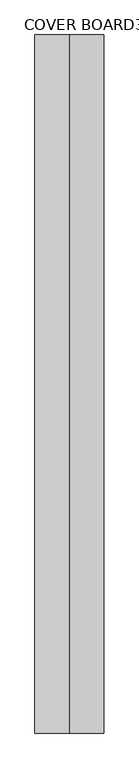
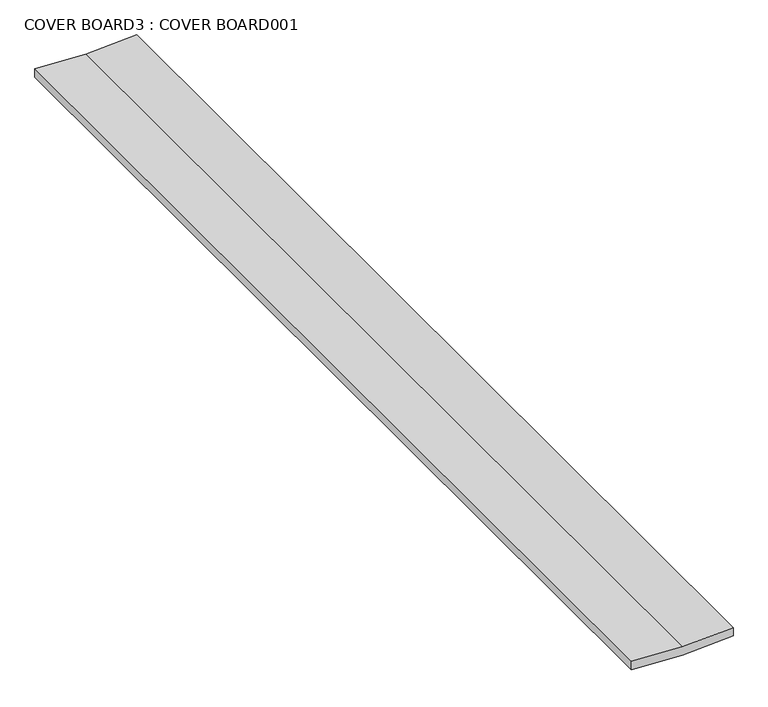
"""IFC4 building model written with IfcOpenShell, lengths in millimetres: proxy geometry, COVER BOARD3 : COVER BOARD001."""

from ifc_helpers import new_model, si_unit, frame, origin, place, context, project, spatial, polyline, outline, extrude, source, transform, mapped, element, save


def cover_board3_cover_board001_2390c736(model_context):
    return source(origin(), model_context, "Body", "SweptSolid", [
        extrude(outline(polyline([(40228.3444286, -4699.8063764), (40233.346, -4797.9038825), (40216.0142809, -4797.9038825), (40211.0127094, -4699.8063764), (40216.0142809, -4601.0538825), (40233.346, -4601.0538825), (40228.3444286, -4699.8063764)])), frame((0.0, -1052.6406573, 0.0), z_axis=(0.0, 1.0, 0.0), x_axis=(0.0, 0.0, 1.0)), (0.0, 0.0, 1.0), 2000.0),
    ])


if __name__ == "__main__":
    model = new_model("IFC4")
    model_context = context("Model", 3, world=origin())
    ifc_project = project(units=[si_unit("LENGTHUNIT", "METRE", prefix="MILLI")], contexts=[model_context])
    site = spatial("IfcSite", under=ifc_project)
    building = spatial("IfcBuilding", under=site)
    placement = place(None, origin())
    cover_board3_cover_board001_shape = cover_board3_cover_board001_2390c736(model_context)
    element("IfcBuildingElementProxy", 1, Name="COVER BOARD3 : COVER BOARD001", ObjectType="COVER BOARD3 : COVER BOARD001", at=placement, inside=building, context=model_context, shape_type="MappedRepresentation", body=[
        mapped(cover_board3_cover_board001_shape, transform((0.0, 0.0, 0.0), x_axis=(1.0, 0.0, 0.0), y_axis=(0.0, 1.0, 0.0), z_axis=(0.0, 0.0, 1.0))),
    ])
    save(model, "model.ifc")

# Revit data of these elements
# Type "COVER BOARD3 : COVER BOARD001"
#   NameOverride = "COVER BOARD001"
# Element 1 (IfcBuildingElementProxy, "COVER BOARD3 : COVER BOARD001")
#   Materials on its faces: "CDX PLYWOOD - SEE STRUCTURAL DWGS"
# Materials
#   "CDX PLYWOOD - SEE STRUCTURAL DWGS": class "Unassigned", colour RGB 202 163 108, transparency 0, Cost = 0
